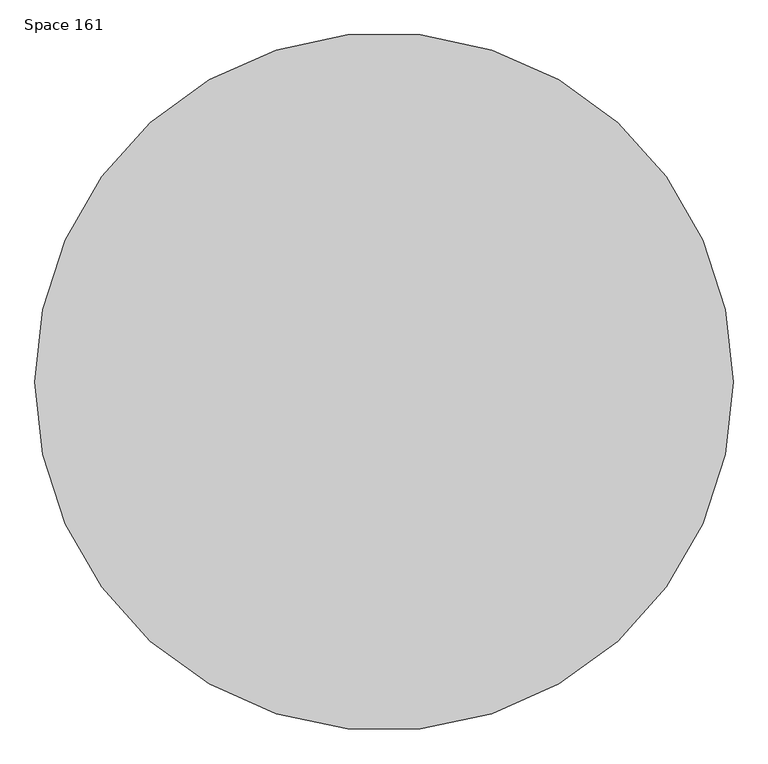
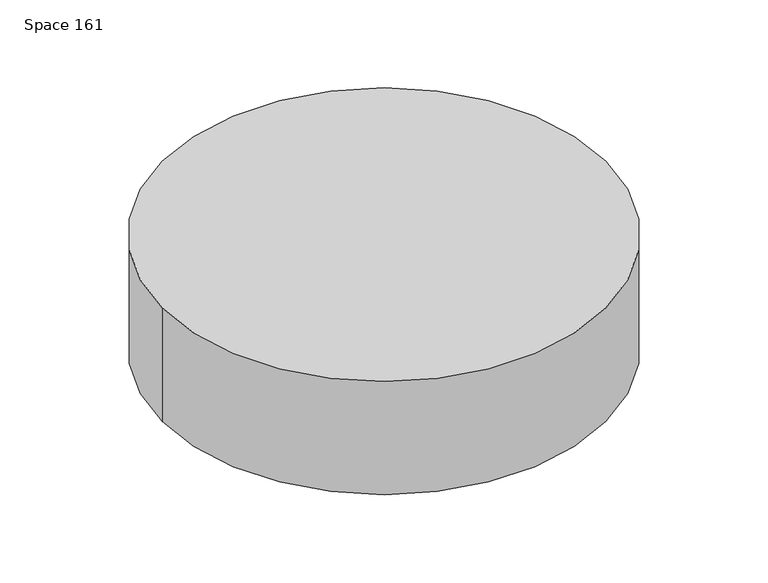
"""IFC4 building model written with IfcOpenShell, lengths in millimetres: proxy geometry, Space 161."""

from ifc_helpers import new_model, si_unit, point, frame, frame_2d, origin, place, context, project, spatial, circle_curve, trimmed, segment, composite_curve, outline, extrude, source, transform, mapped, element, save


def space_161_ce7e7759(model_context):
    return source(origin(), model_context, "Body", "SweptSolid", [
        extrude(outline(composite_curve([segment(trimmed(circle_curve(frame_2d((-24639.5440345, -26167.559635)), 5638.8), [point((-30278.3440345, -26167.559635))], [point((-19000.7440345, -26167.559635))], False, "CARTESIAN"), True, "CONTINUOUS"), segment(trimmed(circle_curve(frame_2d((-24639.5440345, -26167.559635)), 5638.8), [point((-19000.7440345, -26167.559635))], [point((-30278.3440345, -26167.559635))], False, "CARTESIAN"), True, "CONTINUOUS")], self_intersect=False)), frame((0.0, 0.0, 3810.0), z_axis=(0.0, 0.0, 1.0), x_axis=(1.0, 0.0, 0.0)), (0.0, 0.0, 1.0), 3048.0),
    ])


if __name__ == "__main__":
    model = new_model("IFC4")
    model_context = context("Model", 3, world=origin())
    ifc_project = project(units=[si_unit("LENGTHUNIT", "METRE", prefix="MILLI")], contexts=[model_context])
    site = spatial("IfcSite", under=ifc_project)
    building = spatial("IfcBuilding", under=site)
    placement = place(None, origin())
    space_161_shape = space_161_ce7e7759(model_context)
    element("IfcBuildingElementProxy", 1, Name="Space 161", ObjectType="Space 161", at=placement, inside=building, context=model_context, shape_type="MappedRepresentation", body=[
        mapped(space_161_shape, transform((0.0, 0.0, 0.0), x_axis=(1.0, 0.0, 0.0), y_axis=(0.0, 1.0, 0.0), z_axis=(0.0, 0.0, 1.0))),
    ])
    save(model, "model.ifc")

# Revit data of these elements
# Element 1 (IfcBuildingElementProxy, "Space 161")
#   Materials on its faces: "Render Material 255-255-255"
# Materials
#   "Render Material 255-255-255": class "Unassigned", colour RGB 255 255 255, transparency 0
